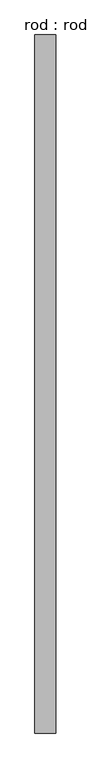
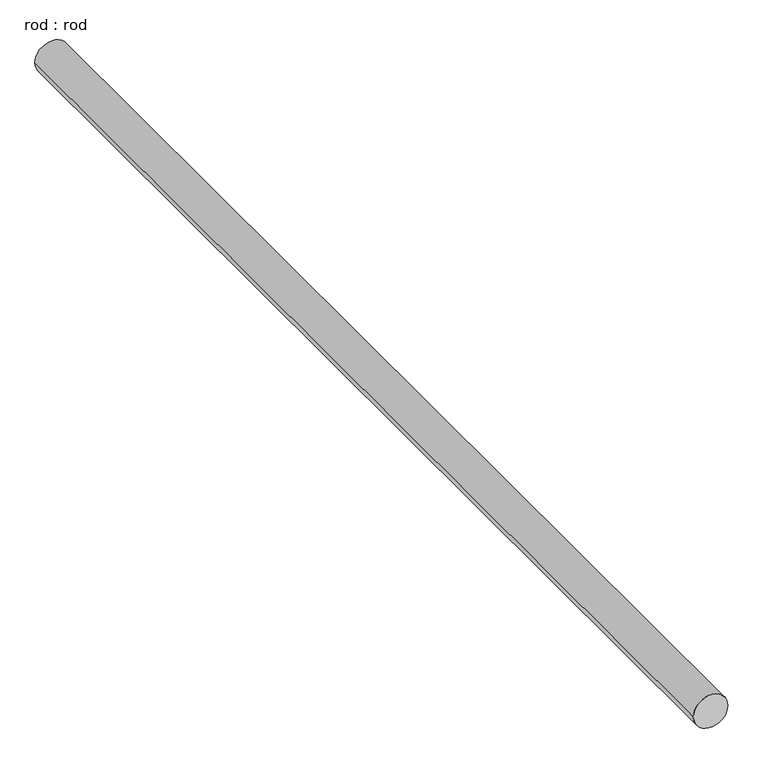
"""IFC4 building model written with IfcOpenShell, lengths in millimetres: proxy geometry, rod : rod."""

from ifc_helpers import new_model, si_unit, point, frame, frame_2d, origin, place, context, project, spatial, circle_curve, trimmed, segment, composite_curve, outline, extrude, source, transform, mapped, element, save


def rod_rod_0f5453ad(model_context):
    return source(origin(), model_context, "Body", "SweptSolid", [
        extrude(outline(composite_curve([segment(trimmed(circle_curve(frame_2d((0.0108462, 0.0)), 200.0), [point((0.0108462, 200.0))], [point((0.0108462, -200.0))], False, "CARTESIAN"), True, "CONTINUOUS"), segment(trimmed(circle_curve(frame_2d((0.0108462, 0.0)), 200.0), [point((0.0108462, -200.0))], [point((0.0108462, 200.0))], False, "CARTESIAN"), True, "CONTINUOUS")], self_intersect=False)), frame((0.0, -2528.12504, 0.0), z_axis=(0.0, 1.0, 0.0), x_axis=(0.0, 0.0, 1.0)), (0.0, 0.0, 1.0), 13241.7073106),
    ])


if __name__ == "__main__":
    model = new_model("IFC4")
    model_context = context("Model", 3, world=origin())
    ifc_project = project(units=[si_unit("LENGTHUNIT", "METRE", prefix="MILLI")], contexts=[model_context])
    site = spatial("IfcSite", under=ifc_project)
    building = spatial("IfcBuilding", under=site)
    placement = place(None, origin())
    rod_rod_shape = rod_rod_0f5453ad(model_context)
    element("IfcBuildingElementProxy", 1, Name="rod : rod", ObjectType="rod : rod", at=placement, inside=building, context=model_context, shape_type="MappedRepresentation", body=[
        mapped(rod_rod_shape, transform((0.0, 0.0, 0.0), x_axis=(1.0, 0.0, 0.0), y_axis=(0.0, 1.0, 0.0), z_axis=(0.0, 0.0, 1.0))),
    ])
    save(model, "model.ifc")

# Revit data of these elements
# Type "rod : rod"
#   Default Elevation = 0
